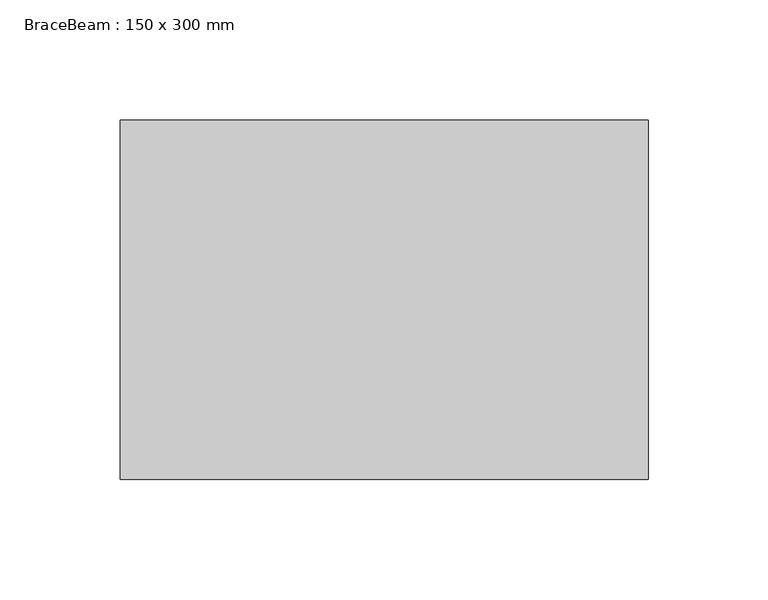
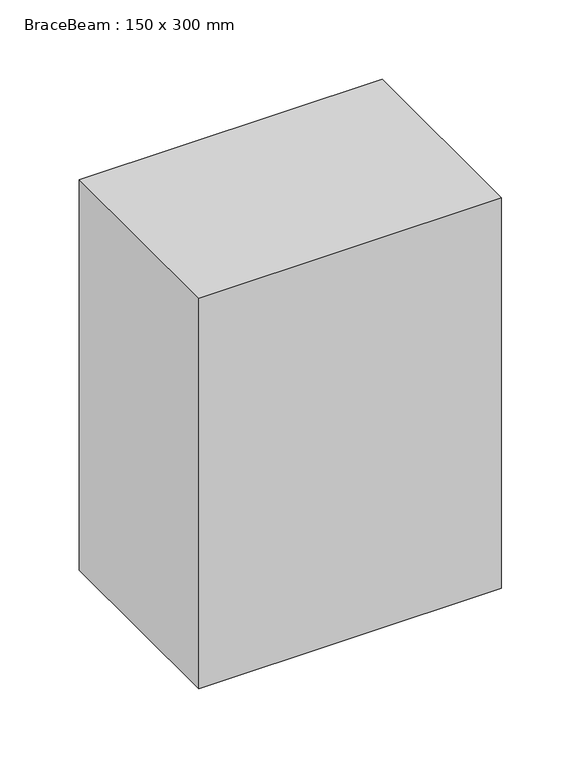
"""IFC4 building model written with IfcOpenShell, lengths in millimetres: beam geometry, BraceBeam : 150 x 300 mm."""

from ifc_helpers import new_model, si_unit, frame, origin, place, context, project, spatial, polyline, outline, extrude, source, transform, mapped, element, save


def bracebeam_150_x_300_mm_8c9a7265(model_context):
    return source(origin(), model_context, "Body", "SweptSolid", [
        extrude(outline(polyline([(-110.0, -75.0), (-110.0, 75.0), (110.0, 75.0), (110.0, -75.0), (-110.0, -75.0)])), frame((0.0, 0.0, -150.0), z_axis=(0.0, 0.0, 1.0), x_axis=(1.0, 0.0, 0.0)), (0.0, 0.0, 1.0), 300.0),
    ])


if __name__ == "__main__":
    model = new_model("IFC4")
    model_context = context("Model", 3, world=origin())
    ifc_project = project(units=[si_unit("LENGTHUNIT", "METRE", prefix="MILLI")], contexts=[model_context])
    site = spatial("IfcSite", under=ifc_project)
    building = spatial("IfcBuilding", under=site)
    placement = place(None, origin())
    bracebeam_150_x_300_mm_shape = bracebeam_150_x_300_mm_8c9a7265(model_context)
    element("IfcBeam", 1, ObjectType="BraceBeam : 150 x 300 mm", at=placement, inside=building, context=model_context, shape_type="MappedRepresentation", body=[
        mapped(bracebeam_150_x_300_mm_shape, transform((0.0, 0.0, 0.0), x_axis=(1.0, 0.0, 0.0), y_axis=(0.0, 1.0, 0.0), z_axis=(0.0, 0.0, 1.0))),
    ])
    save(model, "model.ifc")

# Revit data of these elements
# Type "BraceBeam : 150 x 300 mm"
#   ExpertTruss = "Height\th\r\nWidth\tb"
#   Name [instance default] = ""
#   m [instance default] = 0 mm
#   ip_c_cut_control [instance default] = 1300 mm
#   ip_c_cut [instance default] = 1300 mm
#   h_fix [instance default] = 900 mm
#   d/2 [instance default] = 1750 mm
#   c_cut_incl [instance default] = -1000 mm
#   c_cut [instance default] = 0 mm
#   beta0_2 [instance default] = 90.00°
#   beta0_1 [instance default] = 90.00°
#   alfaMax [instance default] = 0.00°
#   alfa0_2 [instance default] = 90.00°
#   ZOffsetStr_0 [instance default] = 150 mm
#   ZOffsetStr [instance default] = 0 mm
#   ZOffsetEnd_0 [instance default] = 150 mm
#   ZOffsetEnd [instance default] = 0 mm
#   Beta2 [instance default] = 0.00°
#   Beta1 [instance default] = 0.00°
#   Alfa_str [instance default] = 0.00°
#   Alfa_cut_control [instance default] = 90.00°
#   Alfa_cut [instance default] = 90.00°
#   AlfaMAX [instance default] = 0.00°
#   Alfa2_0 [instance default] = 0.00°
#   Alfa2 [instance default] = 0.00°
#   Alfa1_0 [instance default] = 0.00°
#   Alfa1 [instance default] = 0.00°
#   A_max_Str [instance default] = 0.00°
#   h_void [instance default] = 3000 mm
#   beam_L_0 [instance default] = 100 mm
#   beam_L [instance default] = 0 mm
#   b_void [instance default] = 160 mm
#   alfa0_1 [instance default] = 90.00°
#   b = 150 mm
#   YOffsetStr [instance default] = 0 mm
#   YOffsetEnd [instance default] = 0 mm
#   XOffsetStr_0 [instance default] = 3500 mm
#   XOffsetStr [instance default] = 0 mm
#   XOffsetEnd_0 [instance default] = 3500 mm
#   XOffsetEnd [instance default] = 0 mm
#   L_void_0 [instance default] = 100 mm
#   L_void [instance default] = 0 mm
#   E2 [instance default] = 0.00°
#   E1 [instance default] = 0.00°
#   Length [instance default] = 3500 mm
#   h = 300 mm
#   Alfa [instance default] = 0.00°
#   A_max_End [instance default] = 0.00°
#   A_max [instance default] = 0.00°
#   A4 [instance default] = 0.00°
#   A3 [instance default] = 0.00°
#   A2 [instance default] = 0.00°
#   A1 [instance default] = 0.00°
#   BetaAngles [instance default] = no
#   Material [instance default] = Wood Standard
# Element 1 (IfcBeam, "BraceBeam : 150 x 300 mm")
#   d/2 = 185 mm
#   XOffsetStr_0 = 295 mm
#   XOffsetStr = 75 mm
#   XOffsetEnd_0 = 295 mm
#   XOffsetEnd = 75 mm
#   Materials on its faces: "Wood Standard"
# Materials
#   "Wood Standard": class "Drewno", colour RGB 196 146 67, transparency 0, Cost = 0
